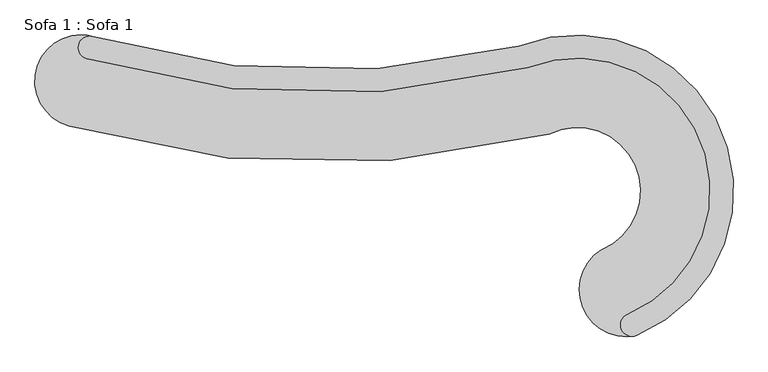
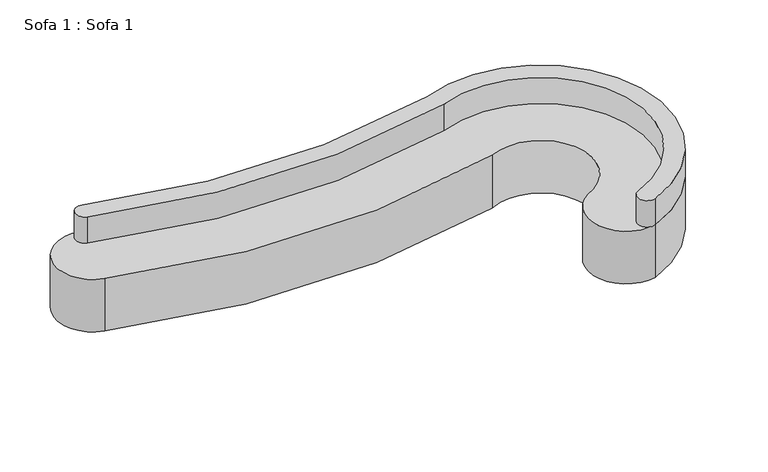
"""IFC4 building model written with IfcOpenShell, lengths in millimetres: furniture geometry, Sofa 1 : Sofa 1."""

from ifc_helpers import new_model, si_unit, point, frame, frame_2d, origin, origin_with_axes, place, context, project, spatial, polyline, circle_curve, trimmed, segment, composite_curve, outline, extrude, source, transform, mapped, element, save
from ifc_brep_helpers import plane_surface, cylinder_surface, revolved_surface, advanced_brep


def sofa_1_sofa_1_ec7ec117(model_context):
    return source(origin(), model_context, "Body", "SolidModel", [
        advanced_brep(
        [(21307.1374885, 18845.8573333, 900.0), (22172.6254157, 16714.9290313, 900.0), (22248.5839685, 16529.9147122, 900.0), (21232.5764018, 19031.4392407, 900.0), (17559.5850592, 19114.9802816, 900.0), (17501.3712996, 18923.6398619, 900.0), (21307.1374885, 18845.8573333, 600.0), (17501.3713025, 18923.6398714, 600.0), (17559.5850592, 19114.9802816, 600.0), (21232.5764018, 19031.4392407, 600.0), (22248.5839685, 16529.9147122, 600.0), (22172.6254157, 16714.9290313, 600.0)],
        [
            (0, 1, circle_curve(frame((21735.863737, 17778.7613658, 900.0), z_axis=(0.0, 0.0, -1.0), x_axis=(0.0, -1.0, 0.0)), 1150.0)),
            (1, 2, circle_curve(frame((22210.6046921, 16622.4218717, 900.0), z_axis=(0.0, 0.0, 1.0), x_axis=(0.0, -1.0, 0.0)), 100.0)),
            (2, 3, circle_curve(frame((21735.863737, 17778.7613658, 900.0), z_axis=(0.0, 0.0, 1.0), x_axis=(0.0, -1.0, 0.0)), 1350.0)),
            (3, 4, circle_curve(frame((19545.6234842, 25648.0529026, 900.0), z_axis=(0.0, 0.0, -1.0), x_axis=(0.0, -1.0, 0.0)), 6828.2784432)),
            (4, 5, circle_curve(frame((17530.4995666, 19019.3035649, 900.0), z_axis=(0.0, 0.0, 1.0), x_axis=(0.0, -1.0, 0.0)), 100.0)),
            (5, 0, circle_curve(frame((19542.0243908, 25625.5981896, 900.0), z_axis=(0.0, 0.0, 1.0), x_axis=(0.0, -1.0, 0.0)), 7005.7483773)),
            (6, 7, circle_curve(frame((19542.0243908, 25625.5981896, 600.0), z_axis=(0.0, 0.0, -1.0), x_axis=(0.0, -1.0, 0.0)), 7005.7483773)),
            (7, 8, circle_curve(frame((17530.4995666, 19019.3035649, 600.0), z_axis=(0.0, 0.0, -1.0), x_axis=(0.0, -1.0, 0.0)), 100.0)),
            (8, 9, circle_curve(frame((19545.6234842, 25648.0529026, 600.0), z_axis=(0.0, 0.0, 1.0), x_axis=(0.0, -1.0, 0.0)), 6828.2784432)),
            (9, 10, circle_curve(frame((21735.863737, 17778.7613658, 600.0), z_axis=(0.0, 0.0, -1.0), x_axis=(0.0, -1.0, 0.0)), 1350.0)),
            (10, 11, circle_curve(frame((22210.6046921, 16622.4218717, 600.0), z_axis=(0.0, 0.0, -1.0), x_axis=(0.0, -1.0, 0.0)), 100.0)),
            (11, 6, circle_curve(frame((21735.863737, 17778.7613658, 600.0), z_axis=(0.0, 0.0, 1.0), x_axis=(0.0, -1.0, 0.0)), 1150.0)),
            (0, 6),
            (11, 1),
            (10, 2),
            (9, 3),
            (8, 4),
            (7, 5),
        ],
        [
            plane_surface(frame((21735.863737, 16628.7613658, 900.0), z_axis=(0.0, 0.0, 1.0), x_axis=(-1.0, 0.0, 0.0))),
            plane_surface(frame((21735.863737, 16628.7613658, 600.0), z_axis=(0.0, 0.0, -1.0), x_axis=(1.0, 0.0, 0.0))),
            revolved_surface(polyline([(21735.863737, 16628.7613658, 600.0), (21735.863737, 16628.7613658, 900.0)]), (21735.863737, 17778.7613658, 600.0), (0.0, 0.0, -1.0)),
            cylinder_surface(frame((22210.6046921, 16622.4218717, 600.0), z_axis=(0.0, 0.0, 1.0), x_axis=(0.0, -1.0, 0.0)), 100.0),
            cylinder_surface(frame((21735.863737, 17778.7613658, 600.0), z_axis=(0.0, 0.0, 1.0), x_axis=(0.0, -1.0, 0.0)), 1350.0),
            revolved_surface(polyline([(19545.6234842, 18819.7744594, 600.0), (19545.6234842, 18819.7744594, 900.0)]), (19545.6234842, 25648.0529026, 600.0), (0.0, 0.0, -1.0)),
            cylinder_surface(frame((17530.4995666, 19019.3035649, 600.0), z_axis=(0.0, 0.0, 1.0), x_axis=(0.0, -1.0, 0.0)), 100.0),
            cylinder_surface(frame((19542.0243908, 25625.5981896, 600.0), z_axis=(0.0, 0.0, 1.0), x_axis=(0.0, -1.0, 0.0)), 7005.7483773),
        ],
        [
            (0, [[1, 2, 3, 4, 5, 6]]),
            (1, [[7, 8, 9, 10, 11, 12]]),
            (2, [[-1, 13, -12, 14]]),
            (3, [[-2, -14, -11, 15]]),
            (4, [[-3, -15, -10, 16]]),
            (5, [[-4, -16, -9, 17]]),
            (6, [[-5, -17, -8, 18]]),
            (7, [[-6, -18, -7, -13]]),
        ],
    ),
        extrude(outline(composite_curve([segment(trimmed(circle_curve(frame_2d((19545.6234842, 25648.0529026)), 7628.2784432), [point((21494.2422379, 18272.8568402))], [point((17352.9346094, 18341.7030955))], False, "CARTESIAN"), True, "CONTINUOUS"), segment(trimmed(circle_curve(frame_2d((17453.874908, 18728.7574277)), 400.0), [point((17352.9346094, 18341.7030955))], [point((17453.8740365, 19128.7574277))], False, "CARTESIAN"), True, "CONTINUOUS"), segment(trimmed(circle_curve(frame_2d((17453.3392525, 18712.2090689)), 416.5487021), [point((17453.8740365, 19128.7574277))], [point((17559.5850592, 19114.9802816))], False, "CARTESIAN"), True, "CONTINUOUS"), segment(trimmed(circle_curve(frame_2d((19545.6234842, 25648.0529026)), 6828.2784432), [point((17559.5850592, 19114.9802816))], [point((21232.5764018, 19031.4392407))], True, "CARTESIAN"), True, "CONTINUOUS"), segment(trimmed(circle_curve(frame_2d((21735.863737, 17778.7613658)), 1350.0), [point((21232.5764018, 19031.4392407))], [point((22248.5839685, 16529.9147122))], False, "CARTESIAN"), True, "CONTINUOUS"), segment(trimmed(circle_curve(frame_2d((22159.4804457, 16925.7317805)), 405.7223057), [point((22248.5839685, 16529.9147122))], [point((21944.7497572, 17269.9719884))], False, "CARTESIAN"), True, "CONTINUOUS"), segment(trimmed(circle_curve(frame_2d((21735.8258248, 17778.7499623)), 550.0038511), [point((21944.7497572, 17269.9719884))], [point((21494.2422379, 18272.8568402))], True, "CARTESIAN"), True, "CONTINUOUS")], self_intersect=False)), origin_with_axes(), (0.0, 0.0, 1.0), 600.0),
    ])


if __name__ == "__main__":
    model = new_model("IFC4")
    model_context = context("Model", 3, world=origin())
    ifc_project = project(units=[si_unit("LENGTHUNIT", "METRE", prefix="MILLI")], contexts=[model_context])
    site = spatial("IfcSite", under=ifc_project)
    building = spatial("IfcBuilding", under=site)
    placement = place(None, origin())
    sofa_1_sofa_1_shape = sofa_1_sofa_1_ec7ec117(model_context)
    element("IfcFurniture", 1, ObjectType="Sofa 1 : Sofa 1", at=placement, inside=building, context=model_context, shape_type="MappedRepresentation", body=[
        mapped(sofa_1_sofa_1_shape, transform((0.0, 0.0, 0.0), x_axis=(1.0, 0.0, 0.0), y_axis=(0.0, 1.0, 0.0), z_axis=(0.0, 0.0, 1.0))),
    ])
    save(model, "model.ifc")

# Revit data of these elements
# Type "Sofa 1 : Sofa 1"
#   Model = "Q1234"
#   Manufacturer = "Irish Seating"
#   Description = "Special edition Sofa"
#   COBie.Type.CreatedBy = "design@eagle.com"
#   COBie.Type.CreatedOn = "2016-09-13T05:47:35"
#   COBie.Type.Name = "Furniture_Sofa 1_Sofa 1"
#   COBie.Type.Category = "23-40 20 14 14 14 : Settees, Sofas"
#   COBie.Type.Description = "Special edition Sofa"
#   COBie.Type.Manufacturer = "Irish Seating"
#   COBie.Type.ModelNumber = "Q1234"
#   COBie.Type.ReplacementCost = 0
#   COBie.Type = yes
